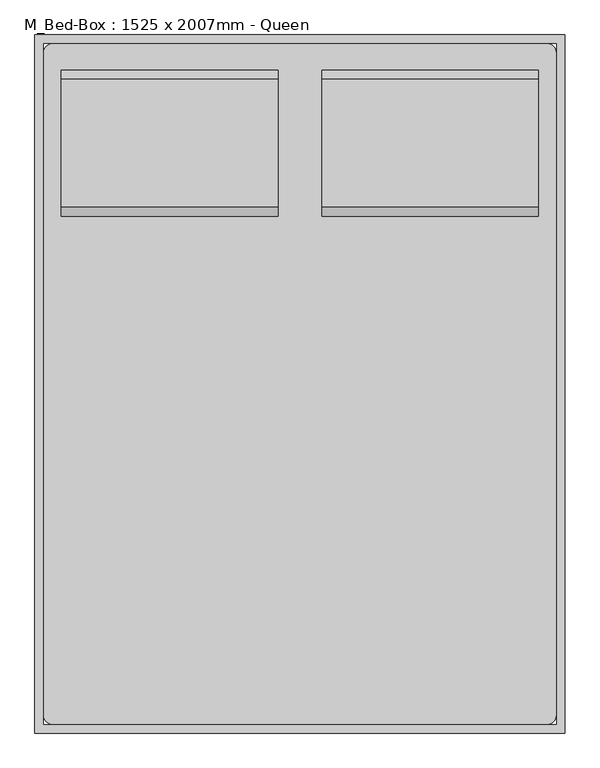
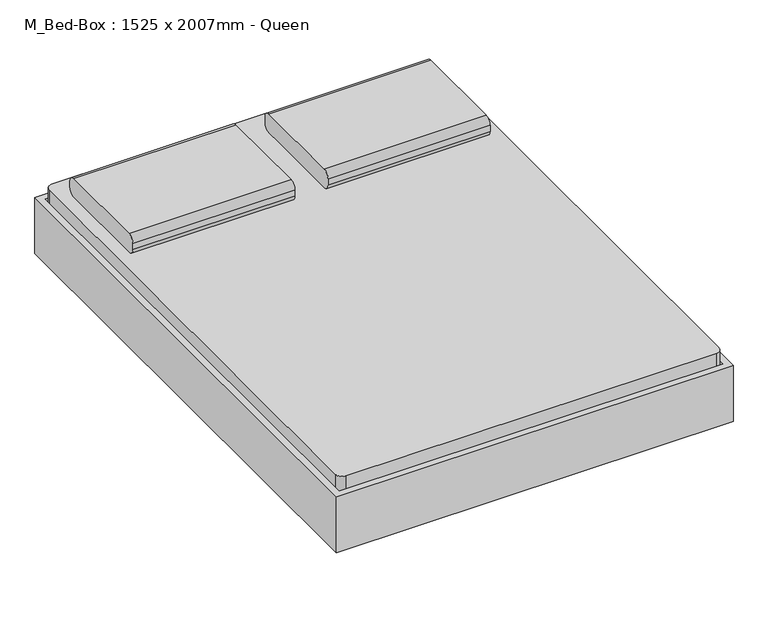
"""IFC4 building model written with IfcOpenShell, lengths in millimetres: furniture geometry, M_Bed-Box : 1525 x 2007mm - Queen."""

import ifcopenshell
import ifcopenshell.guid

model = None  # the IFC model being written
_history = None  # IfcOwnerHistory: only IFC2X3 demands one
_inside = {}  # id of a spatial element -> (the spatial element, [elements in it])
_under = {}  # id of a project, library or spatial element -> (it, [spatial elements below it])
_declared = {}  # id of a project -> (the project, [libraries it declares])
_typed = {}  # id of a type object -> (the type object, [elements of that type])
_made_of = {}  # id of a material, layer set ... -> (it, [elements and type objects made of it])


def new_model(schema):
    """Start an empty IFC model of exactly this schema.

    Asked for "IFC4X3", IfcOpenShell would pick the latest addendum, in which some entities
    have other attributes; the version numbers below select the first issue.
    IFC2X3 requires an IfcOwnerHistory on every rooted entity: one is made here for all.
    """
    global model, _history
    if schema == "IFC4X3":
        model = ifcopenshell.file(schema_version=(4, 3, 0, 0))
    else:
        model = ifcopenshell.file(schema=schema)
    _inside.clear()
    _under.clear()
    _declared.clear()
    _typed.clear()
    _made_of.clear()
    _history = None
    if model.schema == "IFC2X3":
        org = make("IfcOrganization", Name="unknown")
        user = make(
            "IfcPersonAndOrganization",
            ThePerson=make("IfcPerson", FamilyName="unknown"),
            TheOrganization=org,
        )
        app = make(
            "IfcApplication",
            ApplicationDeveloper=org,
            Version="unknown",
            ApplicationFullName="unknown",
            ApplicationIdentifier="unknown",
        )
        _history = make(
            "IfcOwnerHistory",
            OwningUser=user,
            OwningApplication=app,
            ChangeAction="ADDED",
            CreationDate=0,
        )
    return model


def make(cls, **values):
    """One entity of the class cls with the attributes given. An attribute that is None is left unset."""
    return model.create_entity(
        cls, **{name: value for name, value in values.items() if value is not None}
    )


def rooted(cls, **values):
    """An entity with a GlobalId (a new one), such as an element, a storey or a relation."""
    return make(cls, GlobalId=ifcopenshell.guid.new(), OwnerHistory=_history, **values)


def si_unit(unit_type, name, prefix=None):
    """IfcSIUnit, for example si_unit("LENGTHUNIT", "METRE", prefix="MILLI")."""
    return make("IfcSIUnit", UnitType=unit_type, Prefix=prefix, Name=name)


def assignment(units):
    """IfcUnitAssignment: the units of a project."""
    return None if units is None else make("IfcUnitAssignment", Units=units)


def point(xyz):
    """IfcCartesianPoint."""
    return None if xyz is None else make("IfcCartesianPoint", Coordinates=xyz)


def direction(xyz):
    """IfcDirection."""
    return None if xyz is None else make("IfcDirection", DirectionRatios=xyz)


def frame(location, z_axis=None, x_axis=None):
    """IfcAxis2Placement3D, a coordinate frame: its origin and axes. An axis left out is left unset."""
    return make(
        "IfcAxis2Placement3D",
        Location=point(location),
        Axis=direction(z_axis),
        RefDirection=direction(x_axis),
    )


def frame_2d(location, x_axis=None):
    """IfcAxis2Placement2D, a coordinate frame in the plane: its origin and x axis."""
    return make(
        "IfcAxis2Placement2D", Location=point(location), RefDirection=direction(x_axis)
    )


def origin():
    """The frame at (0, 0, 0) with its axes left unset."""
    return frame((0.0, 0.0, 0.0))


def place(relative_to, where):
    """IfcLocalPlacement: puts the frame where relative to a parent placement (None: the world)."""
    return make(
        "IfcLocalPlacement", PlacementRelTo=relative_to, RelativePlacement=where
    )


def context(
    kind, dimensions, precision=None, world=None, true_north=None, identifier=None
):
    """IfcGeometricRepresentationContext, for example the 3D "Model" context."""
    return make(
        "IfcGeometricRepresentationContext",
        ContextIdentifier=identifier,
        ContextType=kind,
        CoordinateSpaceDimension=dimensions,
        Precision=precision,
        WorldCoordinateSystem=world,
        TrueNorth=true_north,
    )


def project(units=None, contexts=None):
    """IfcProject with its units and contexts."""
    return rooted(
        "IfcProject",
        Name="project",
        RepresentationContexts=contexts,
        UnitsInContext=assignment(units),
    )


def spatial(cls, under=None, at=None, **own):
    """A site, building, storey or space (cls), placed at a placement, below another one or the project."""
    s = rooted(cls, ObjectPlacement=at, **own)
    if under is not None:
        _under.setdefault(under.id(), (under, []))[1].append(s)
    return s


def polyline(points):
    """IfcPolyline through the points."""
    return make("IfcPolyline", Points=[point(p) for p in points])


def circle_curve(where, radius):
    """IfcCircle in the frame where."""
    return make("IfcCircle", Position=where, Radius=radius)


def trimmed(basis, trim1, trim2, sense, master):
    """IfcTrimmedCurve: the piece of a basis curve between two trims."""
    return make(
        "IfcTrimmedCurve",
        BasisCurve=basis,
        Trim1=trim1,
        Trim2=trim2,
        SenseAgreement=sense,
        MasterRepresentation=master,
    )


def segment(curve, same_sense, transition):
    """IfcCompositeCurveSegment."""
    return make(
        "IfcCompositeCurveSegment",
        Transition=transition,
        SameSense=same_sense,
        ParentCurve=curve,
    )


def composite_curve(segments, self_intersect=None):
    """IfcCompositeCurve: segments joined end to end."""
    return make("IfcCompositeCurve", Segments=segments, SelfIntersect=self_intersect)


def outline(outer, holes=None, kind="AREA"):
    """IfcArbitraryClosedProfileDef: a profile drawn as a closed curve; with holes, ...WithVoids."""
    if holes is None:
        return make("IfcArbitraryClosedProfileDef", ProfileType=kind, OuterCurve=outer)
    return make(
        "IfcArbitraryProfileDefWithVoids",
        ProfileType=kind,
        OuterCurve=outer,
        InnerCurves=holes,
    )


def extrude(swept, where, along, depth):
    """IfcExtrudedAreaSolid: the profile swept, set in the frame where, extruded along a direction by depth."""
    return make(
        "IfcExtrudedAreaSolid",
        SweptArea=swept,
        Position=where,
        ExtrudedDirection=direction(along),
        Depth=depth,
    )


def shape(context_of_items, identifier, shape_type, items):
    """IfcShapeRepresentation: the items that make up one representation, for example the "Body"."""
    return make(
        "IfcShapeRepresentation",
        ContextOfItems=context_of_items,
        RepresentationIdentifier=identifier,
        RepresentationType=shape_type,
        Items=items,
    )


def source(mapping_origin, context_of_items, identifier, shape_type, items):
    """IfcRepresentationMap: a shape defined once, which mapped items show again and again."""
    return make(
        "IfcRepresentationMap",
        MappingOrigin=mapping_origin,
        MappedRepresentation=shape(context_of_items, identifier, shape_type, items),
    )


def transform(
    local_origin,
    x_axis=None,
    y_axis=None,
    z_axis=None,
    scale=None,
    scale2=None,
    scale3=None,
    uniform=True,
):
    """IfcCartesianTransformationOperator3D, or its non-uniform kind. x_axis, y_axis, z_axis: its Axis1, 2, 3."""
    if uniform:
        return make(
            "IfcCartesianTransformationOperator3D",
            Axis1=direction(x_axis),
            Axis2=direction(y_axis),
            LocalOrigin=point(local_origin),
            Scale=scale,
            Axis3=direction(z_axis),
        )
    return make(
        "IfcCartesianTransformationOperator3DnonUniform",
        Axis1=direction(x_axis),
        Axis2=direction(y_axis),
        LocalOrigin=point(local_origin),
        Scale=scale,
        Axis3=direction(z_axis),
        Scale2=scale2,
        Scale3=scale3,
    )


def mapped(mapping_source, mapping_target):
    """IfcMappedItem: shows the shape of a source again, moved by a transform."""
    return make(
        "IfcMappedItem", MappingSource=mapping_source, MappingTarget=mapping_target
    )


def made_of(thing, what):
    """Note that an element or type object is made of a material, layer set ...; save() writes the relation."""
    if what is not None:
        _made_of.setdefault(what.id(), (what, []))[1].append(thing)
    return thing


def element(
    cls,
    number,
    at=None,
    inside=None,
    cuts=None,
    type_object=None,
    material=None,
    context=None,
    identifier="Body",
    shape_type=None,
    held_by="IfcProductDefinitionShape",
    body=None,
    shapes=None,
    **own,
):
    """One element of the class cls, such as IfcWall. Its Tag is "e" and its number.

    at: its placement. inside: the storey or other place that contains it. cuts: it is an
    opening in that element (IfcRelVoidsElement). A single representation is given by context,
    identifier, shape_type and body (its items); several are given by shapes. held_by: the class
    of the entity that holds the representations. save() writes the other relations.
    """
    e = rooted(cls, Tag="e%d" % number, ObjectPlacement=at, **own)
    if body is not None:
        shapes = [shape(context, identifier, shape_type, body)]
    if shapes is not None:
        e.Representation = make(held_by, Representations=shapes)
    if inside is not None:
        _inside.setdefault(inside.id(), (inside, []))[1].append(e)
    if cuts is not None:
        rooted(
            "IfcRelVoidsElement", RelatingBuildingElement=cuts, RelatedOpeningElement=e
        )
    if type_object is not None:
        _typed.setdefault(type_object.id(), (type_object, []))[1].append(e)
    return made_of(e, material)


def aggregate(whole, parts):
    """IfcRelAggregates: a whole, such as a stair, and the parts it consists of."""
    return rooted("IfcRelAggregates", RelatingObject=whole, RelatedObjects=parts)


def save(model, path):
    """Write the relations noted so far, then the file.

    IfcRelAggregates (storeys below a building ...), IfcRelContainedInSpatialStructure (elements
    in a storey), IfcRelDefinesByType, IfcRelAssociatesMaterial and IfcRelDeclares: one each for
    every whole, place, type object, material and project.
    """
    for whole, parts in _under.values():
        aggregate(whole, parts)
    for where, things in _inside.values():
        rooted(
            "IfcRelContainedInSpatialStructure",
            RelatedElements=things,
            RelatingStructure=where,
        )
    for kind, things in _typed.values():
        rooted("IfcRelDefinesByType", RelatedObjects=things, RelatingType=kind)
    for what, things in _made_of.values():
        rooted("IfcRelAssociatesMaterial", RelatedObjects=things, RelatingMaterial=what)
    for by, libraries in _declared.values():
        rooted("IfcRelDeclares", RelatingContext=by, RelatedDefinitions=libraries)
    model.write(path)


def plane_surface(at):
    """IfcPlane: the flat surface through the origin of the frame at, square to its z axis."""
    return make("IfcPlane", Position=at)


def cylinder_surface(at, radius):
    """IfcCylindricalSurface: all points at the distance radius from the z axis of the frame at."""
    return make("IfcCylindricalSurface", Position=at, Radius=radius)


def revolved_surface(curve, axis_point, axis_direction):
    """IfcSurfaceOfRevolution: the curve turned about the line through axis_point along axis_direction."""
    return make(
        "IfcSurfaceOfRevolution",
        SweptCurve=make("IfcArbitraryOpenProfileDef", ProfileType="CURVE", Curve=curve),
        AxisPosition=make("IfcAxis1Placement", Location=point(axis_point), Axis=direction(axis_direction)),
    )


def advanced_brep(points, edges, surfaces, faces):
    """IfcAdvancedBrep: a solid bounded by faces that lie on surfaces and meet in shared edges.

    An edge is (start, end): straight between two places in points (the first is 0);
    or (start, end, curve); or (start, end, curve, False) where it runs against its curve.
    A face is (place in surfaces, loops), or (place, loops, False) where it looks against
    its surface's normal. A loop lists edges by number (the first is 1), with a minus sign
    where the edge is run from its end to its start. The first loop is the outer one.
    """
    corners = [point(p) for p in points]
    vertices = [make("IfcVertexPoint", VertexGeometry=c) for c in corners]
    made = []
    for start, end, *more in edges:
        made.append(
            make(
                "IfcEdgeCurve",
                EdgeStart=vertices[start],
                EdgeEnd=vertices[end],
                EdgeGeometry=more[0] if more else make("IfcPolyline", Points=[corners[start], corners[end]]),
                SameSense=more[1] if len(more) > 1 else True,
            )
        )
    hull = []
    for where, loops, *sense in faces:
        bounds = []
        for j, loop in enumerate(loops):
            ring = [make("IfcOrientedEdge", EdgeElement=made[abs(k) - 1], Orientation=k > 0) for k in loop]
            bounds.append(
                make(
                    "IfcFaceOuterBound" if j == 0 else "IfcFaceBound",
                    Bound=make("IfcEdgeLoop", EdgeList=ring),
                    Orientation=True,
                )
            )
        hull.append(make("IfcAdvancedFace", Bounds=bounds, FaceSurface=surfaces[where], SameSense=sense[0] if sense else True))
    return make("IfcAdvancedBrep", Outer=make("IfcClosedShell", CfsFaces=hull))


def m_bed_box_1525_x_2007mm_queen_e2603687(model_context):
    return source(origin(), model_context, "Body", "SolidModel", [
        extrude(outline(composite_curve([segment(polyline([(642.0704918, 406.4), (273.7704918, 406.4)]), True, "CONTINUOUS"), segment(trimmed(circle_curve(frame_2d((273.7704918, 431.8)), 25.4), [point((273.7704918, 406.4))], [point((248.3704918, 431.8))], False, "CARTESIAN"), True, "CONTINUOUS"), segment(polyline([(248.3704918, 431.8), (248.3704918, 457.2)]), True, "CONTINUOUS"), segment(trimmed(circle_curve(frame_2d((273.7704918, 457.2)), 25.4), [point((248.3704918, 457.2))], [point((273.7704918, 482.6))], False, "CARTESIAN"), True, "CONTINUOUS"), segment(polyline([(273.7704918, 482.6), (642.0704918, 482.6)]), True, "CONTINUOUS"), segment(trimmed(circle_curve(frame_2d((642.0704918, 457.2)), 25.4), [point((642.0704918, 482.6))], [point((667.4704918, 457.2))], False, "CARTESIAN"), True, "CONTINUOUS"), segment(polyline([(667.4704918, 457.2), (667.4704918, 431.8)]), True, "CONTINUOUS"), segment(trimmed(circle_curve(frame_2d((642.0704918, 431.8)), 25.4), [point((667.4704918, 431.8))], [point((642.0704918, 406.4))], False, "CARTESIAN"), True, "CONTINUOUS")], self_intersect=False)), frame((402.652459, 0.0, 0.0), z_axis=(1.0, 0.0, 0.0), x_axis=(0.0, 1.0, 0.0)), (0.0, 0.0, 1.0), 622.8),
        extrude(outline(composite_curve([segment(polyline([(642.0704918, 406.4), (273.7704918, 406.4)]), True, "CONTINUOUS"), segment(trimmed(circle_curve(frame_2d((273.7704918, 431.8)), 25.4), [point((273.7704918, 406.4))], [point((248.3704918, 431.8))], False, "CARTESIAN"), True, "CONTINUOUS"), segment(polyline([(248.3704918, 431.8), (248.3704918, 457.2)]), True, "CONTINUOUS"), segment(trimmed(circle_curve(frame_2d((273.7704918, 457.2)), 25.4), [point((248.3704918, 457.2))], [point((273.7704918, 482.6))], False, "CARTESIAN"), True, "CONTINUOUS"), segment(polyline([(273.7704918, 482.6), (642.0704918, 482.6)]), True, "CONTINUOUS"), segment(trimmed(circle_curve(frame_2d((642.0704918, 457.2)), 25.4), [point((642.0704918, 482.6))], [point((667.4704918, 457.2))], False, "CARTESIAN"), True, "CONTINUOUS"), segment(polyline([(667.4704918, 457.2), (667.4704918, 431.8)]), True, "CONTINUOUS"), segment(trimmed(circle_curve(frame_2d((642.0704918, 431.8)), 25.4), [point((667.4704918, 431.8))], [point((642.0704918, 406.4))], False, "CARTESIAN"), True, "CONTINUOUS")], self_intersect=False)), frame((-347.147541, 0.0, 0.0), z_axis=(1.0, 0.0, 0.0), x_axis=(0.0, 1.0, 0.0)), (0.0, 0.0, 1.0), 622.8),
        advanced_brep(
        [(-397.6231784, 515.0704918, 177.8), (-397.6231784, 438.8704918, 177.8), (-397.6231784, 438.8704918, 196.85), (-397.6231784, 515.0704918, 196.85), (-346.8231784, 515.0704918, 177.8), (-346.8231784, 438.8704918, 177.8), (-334.6869899, 438.8704918, 196.85), (-334.6869899, 515.0704918, 196.85), (-270.7523099, 515.0704918, 14.6654962), (-270.7523099, 438.8704918, 14.6654962), (-253.4871466, 438.8704918, 22.716374), (-253.4871466, 515.0704918, 22.716374), (-247.7320921, 438.8704918, 0.0), (-247.7320921, 515.0704918, 0.0), (-247.7320921, 438.8704918, 19.05), (-247.7320921, 515.0704918, 19.05), (-169.1195862, 515.0704918, 0.0), (-169.1195862, 438.8704918, 0.0), (-169.1195862, 438.8704918, 19.05), (-169.1195862, 515.0704918, 19.05), (-156.4195862, 438.8704918, 3.4029547), (-156.4195862, 515.0704918, 3.4029547), (-165.9445862, 438.8704918, 19.9007387), (-165.9445862, 515.0704918, 19.9007387), (-96.322541, 515.0704918, 38.1), (-96.322541, 438.8704918, 38.1), (-101.4269731, 438.8704918, 57.15), (-101.4269731, 515.0704918, 57.15), (774.9518216, 515.0704918, 38.1), (774.9518216, 438.8704918, 38.1), (780.0562537, 438.8704918, 57.15), (780.0562537, 515.0704918, 57.15), (835.0488669, 515.0704918, 3.4029547), (835.0488669, 438.8704918, 3.4029547), (844.5738669, 438.8704918, 19.9007387), (844.5738669, 515.0704918, 19.9007387), (847.7488669, 438.8704918, 0.0), (847.7488669, 515.0704918, 0.0), (847.7488669, 438.8704918, 19.05), (847.7488669, 515.0704918, 19.05), (926.3613728, 515.0704918, 0.0), (926.3613728, 438.8704918, 0.0), (926.3613728, 438.8704918, 19.05), (926.3613728, 515.0704918, 19.05), (949.3815906, 438.8704918, 14.6654962), (949.3815906, 515.0704918, 14.6654962), (932.1164272, 438.8704918, 22.716374), (932.1164272, 515.0704918, 22.716374), (1025.452459, 515.0704918, 177.8), (1025.452459, 438.8704918, 177.8), (1013.3162705, 438.8704918, 196.85), (1013.3162705, 515.0704918, 196.85), (1076.252459, 515.0704918, 177.8), (1076.252459, 515.0704918, 196.85), (1076.252459, 438.8704918, 196.85), (1076.252459, 438.8704918, 177.8)],
        [
            (0, 1),
            (1, 2),
            (2, 3),
            (3, 0),
            (0, 4),
            (4, 5),
            (5, 1),
            (5, 6),
            (6, 2),
            (6, 7),
            (7, 3),
            (7, 4),
            (4, 8),
            (8, 9),
            (9, 5),
            (9, 10),
            (10, 6),
            (10, 11),
            (11, 7),
            (11, 8),
            (12, 9, circle_curve(frame((-247.7320921, 438.8704918, 25.4), z_axis=(0.0, 1.0, 0.0), x_axis=(-0.906307787036649, 0.0, -0.4226182617407015)), 25.4)),
            (8, 13, circle_curve(frame((-247.7320921, 515.0704918, 25.4), z_axis=(0.0, -1.0, 0.0), x_axis=(-0.906307787036649, 0.0, -0.4226182617407015)), 25.4)),
            (13, 12),
            (14, 10, circle_curve(frame((-247.7320921, 438.8704918, 25.4), z_axis=(0.0, 1.0, 0.0), x_axis=(-0.906307787036649, 0.0, -0.4226182617407015)), 6.35)),
            (12, 14),
            (15, 11, circle_curve(frame((-247.7320921, 515.0704918, 25.4), z_axis=(0.0, 1.0, 0.0), x_axis=(-0.906307787036649, 0.0, -0.4226182617407015)), 6.35)),
            (14, 15),
            (15, 13),
            (13, 16),
            (16, 17),
            (17, 12),
            (17, 18),
            (18, 14),
            (18, 19),
            (19, 15),
            (19, 16),
            (20, 17, circle_curve(frame((-169.1195862, 438.8704918, 25.4), z_axis=(0.0, 1.0, 0.0), x_axis=(0.0, 0.0, -1.0)), 25.4)),
            (16, 21, circle_curve(frame((-169.1195862, 515.0704918, 25.4), z_axis=(0.0, -1.0, 0.0), x_axis=(0.0, 0.0, -1.0)), 25.4)),
            (21, 20),
            (22, 18, circle_curve(frame((-169.1195862, 438.8704918, 25.4), z_axis=(0.0, 1.0, 0.0), x_axis=(0.0, 0.0, -1.0)), 6.35)),
            (20, 22),
            (23, 19, circle_curve(frame((-169.1195862, 515.0704918, 25.4), z_axis=(0.0, 1.0, 0.0), x_axis=(0.0, 0.0, -1.0)), 6.35)),
            (22, 23),
            (23, 21),
            (21, 24),
            (24, 25),
            (25, 20),
            (25, 26),
            (26, 22),
            (26, 27),
            (27, 23),
            (27, 24),
            (24, 28),
            (28, 29),
            (29, 25),
            (29, 30),
            (30, 26),
            (30, 31),
            (31, 27),
            (31, 28),
            (28, 32),
            (32, 33),
            (33, 29),
            (33, 34),
            (34, 30),
            (34, 35),
            (35, 31),
            (35, 32),
            (36, 33, circle_curve(frame((847.7488669, 438.8704918, 25.4), z_axis=(0.0, 1.0, 0.0), x_axis=(-0.5000000000000463, 0.0, -0.8660254037844118)), 25.4)),
            (32, 37, circle_curve(frame((847.7488669, 515.0704918, 25.4), z_axis=(0.0, -1.0, 0.0), x_axis=(-0.5000000000000463, 0.0, -0.8660254037844118)), 25.4)),
            (37, 36),
            (38, 34, circle_curve(frame((847.7488669, 438.8704918, 25.4), z_axis=(0.0, 1.0, 0.0), x_axis=(-0.5000000000000463, 0.0, -0.8660254037844118)), 6.35)),
            (36, 38),
            (39, 35, circle_curve(frame((847.7488669, 515.0704918, 25.4), z_axis=(0.0, 1.0, 0.0), x_axis=(-0.5000000000000463, 0.0, -0.8660254037844118)), 6.35)),
            (38, 39),
            (39, 37),
            (37, 40),
            (40, 41),
            (41, 36),
            (41, 42),
            (42, 38),
            (42, 43),
            (43, 39),
            (43, 40),
            (44, 41, circle_curve(frame((926.3613728, 438.8704918, 25.4), z_axis=(0.0, 1.0, 0.0), x_axis=(0.0, 0.0, -1.0)), 25.4)),
            (40, 45, circle_curve(frame((926.3613728, 515.0704918, 25.4), z_axis=(0.0, -1.0, 0.0), x_axis=(0.0, 0.0, -1.0)), 25.4)),
            (45, 44),
            (46, 42, circle_curve(frame((926.3613728, 438.8704918, 25.4), z_axis=(0.0, 1.0, 0.0), x_axis=(0.0, 0.0, -1.0)), 6.35)),
            (44, 46),
            (47, 43, circle_curve(frame((926.3613728, 515.0704918, 25.4), z_axis=(0.0, 1.0, 0.0), x_axis=(0.0, 0.0, -1.0)), 6.35)),
            (46, 47),
            (47, 45),
            (45, 48),
            (48, 49),
            (49, 44),
            (49, 50),
            (50, 46),
            (50, 51),
            (51, 47),
            (51, 48),
            (52, 53),
            (53, 54),
            (54, 55),
            (55, 52),
            (48, 52),
            (55, 49),
            (54, 50),
            (53, 51),
        ],
        [
            plane_surface(frame((-397.6231784, 769.0704918, -152.9490627), z_axis=(-1.0, 0.0, 0.0), x_axis=(0.0, 1.0, 0.0))),
            plane_surface(frame((-397.6231784, 515.0704918, 177.8), z_axis=(0.0, 0.0, -1.0), x_axis=(1.0, 0.0, 0.0))),
            plane_surface(frame((-397.6231784, 438.8704918, 177.8), z_axis=(0.0, -1.0, 0.0), x_axis=(1.0, 0.0, 0.0))),
            plane_surface(frame((-397.6231784, 438.8704918, 196.85), z_axis=(0.0, 0.0, 1.0), x_axis=(1.0, 0.0, 0.0))),
            plane_surface(frame((-397.6231784, 515.0704918, 196.85), z_axis=(0.0, 1.0, 0.0), x_axis=(1.0, 0.0, 0.0))),
            plane_surface(frame((-346.8231784, 515.0704918, 177.8), z_axis=(-0.9063077870366485, 0.0, -0.4226182617407029), x_axis=(0.4226182617407029, 0.0, -0.9063077870366485))),
            plane_surface(frame((-346.8231784, 438.8704918, 177.8), z_axis=(0.0, -1.0, 0.0), x_axis=(0.42261826174070266, 0.0, -0.9063077870366485))),
            plane_surface(frame((-334.6869899, 438.8704918, 196.85), z_axis=(0.9063077870366486, 0.0, 0.4226182617407026), x_axis=(0.4226182617407026, 0.0, -0.9063077870366486))),
            plane_surface(frame((-334.6869899, 515.0704918, 196.85), z_axis=(0.0, 1.0, 0.0), x_axis=(0.42261826174070266, 0.0, -0.9063077870366485))),
            cylinder_surface(frame((-247.7320921, 769.0704918, 25.4), z_axis=(0.0, -1.0, 0.0), x_axis=(-0.906307787036649, 0.0, -0.4226182617407015)), 25.4),
            plane_surface(frame((-247.7320921, 438.8704918, 25.4), z_axis=(0.0, -1.0, 0.0), x_axis=(-0.906307787036649, 0.0, -0.4226182617407015))),
            revolved_surface(polyline([(-253.4871465476827, 438.8704918, 22.716374037946544), (-253.4871465476827, 515.0704918, 22.716374037946544)]), (-247.7320921, 769.0704918, 25.4), (0.0, -1.0, 0.0)),
            plane_surface(frame((-247.7320921, 515.0704918, 25.4), z_axis=(0.0, 1.0, 0.0), x_axis=(-0.906307787036649, 0.0, -0.4226182617407015))),
            plane_surface(frame((-247.7320921, 515.0704918, 0.0), z_axis=(0.0, 0.0, -1.0), x_axis=(1.0, 0.0, 0.0))),
            plane_surface(frame((-247.7320921, 438.8704918, 0.0), z_axis=(0.0, -1.0, 0.0), x_axis=(1.0, 0.0, 0.0))),
            plane_surface(frame((-247.7320921, 438.8704918, 19.05), z_axis=(0.0, 0.0, 1.0), x_axis=(1.0, 0.0, 0.0))),
            plane_surface(frame((-247.7320921, 515.0704918, 19.05), z_axis=(0.0, 1.0, 0.0), x_axis=(1.0, 0.0, 0.0))),
            cylinder_surface(frame((-169.1195862, 769.0704918, 25.4), z_axis=(0.0, -1.0, 0.0), x_axis=(0.0, 0.0, -1.0)), 25.4),
            plane_surface(frame((-169.1195862, 438.8704918, 25.4), z_axis=(0.0, -1.0, 0.0), x_axis=(0.0, 0.0, -1.0))),
            revolved_surface(polyline([(-169.1195862, 438.8704918, 19.049999999999997), (-169.1195862, 515.0704918, 19.049999999999997)]), (-169.1195862, 769.0704918, 25.4), (0.0, -1.0, 0.0)),
            plane_surface(frame((-169.1195862, 515.0704918, 25.4), z_axis=(0.0, 1.0, 0.0), x_axis=(0.0, 0.0, -1.0))),
            plane_surface(frame((-156.4195862, 515.0704918, 3.4029547), z_axis=(0.49999999999987765, 0.0, -0.8660254037845093), x_axis=(0.8660254037845093, 0.0, 0.49999999999987765))),
            plane_surface(frame((-156.4195862, 438.8704918, 3.4029547), z_axis=(0.0, -1.0, 0.0), x_axis=(0.8660254037845091, 0.0, 0.499999999999878))),
            plane_surface(frame((-165.9445862, 438.8704918, 19.9007387), z_axis=(-0.49999999999987765, 0.0, 0.8660254037845093), x_axis=(0.8660254037845093, 0.0, 0.49999999999987765))),
            plane_surface(frame((-165.9445862, 515.0704918, 19.9007387), z_axis=(0.0, 1.0000000000000002, 0.0), x_axis=(0.8660254037845089, 0.0, 0.4999999999998785))),
            plane_surface(frame((-96.322541, 515.0704918, 38.1), z_axis=(0.0, 0.0, -1.0), x_axis=(1.0, 0.0, 0.0))),
            plane_surface(frame((-96.322541, 438.8704918, 38.1), z_axis=(0.0, -1.0, 0.0), x_axis=(1.0, 0.0, 0.0))),
            plane_surface(frame((-101.4269731, 438.8704918, 57.15), z_axis=(0.0, 0.0, 1.0), x_axis=(1.0, 0.0, 0.0))),
            plane_surface(frame((-101.4269731, 515.0704918, 57.15), z_axis=(0.0, 1.0, 0.0), x_axis=(1.0, 0.0, 0.0))),
            plane_surface(frame((774.9518216, 515.0704918, 38.1), z_axis=(-0.5000000000000452, 0.0, -0.8660254037844126), x_axis=(0.8660254037844126, 0.0, -0.5000000000000452))),
            plane_surface(frame((774.9518216, 438.8704918, 38.1), z_axis=(0.0, -1.0, 0.0), x_axis=(0.8660254037844124, 0.0, -0.5000000000000455))),
            plane_surface(frame((780.0562537, 438.8704918, 57.15), z_axis=(0.5000000000000464, 0.0, 0.8660254037844118), x_axis=(0.8660254037844118, 0.0, -0.5000000000000464))),
            plane_surface(frame((780.0562537, 515.0704918, 57.15), z_axis=(0.0, 1.0000000000000002, 0.0), x_axis=(0.866025403784413, 0.0, -0.5000000000000447))),
            cylinder_surface(frame((847.7488669, 769.0704918, 25.4), z_axis=(0.0, -1.0, 0.0), x_axis=(-0.5000000000000463, 0.0, -0.8660254037844118)), 25.4),
            plane_surface(frame((847.7488669, 438.8704918, 25.4), z_axis=(0.0, -1.0000000000000002, 0.0), x_axis=(-0.5000000000000464, 0.0, -0.866025403784412))),
            revolved_surface(polyline([(844.5738668999998, 438.8704918, 19.90073868596898), (844.5738668999998, 515.0704918, 19.90073868596898)]), (847.7488669, 769.0704918, 25.4), (0.0, -1.0, 0.0)),
            plane_surface(frame((847.7488669, 515.0704918, 25.4), z_axis=(0.0, 1.0000000000000002, 0.0), x_axis=(-0.5000000000000464, 0.0, -0.866025403784412))),
            plane_surface(frame((847.7488669, 515.0704918, 0.0), z_axis=(0.0, 0.0, -1.0), x_axis=(1.0, 0.0, 0.0))),
            plane_surface(frame((847.7488669, 438.8704918, 0.0), z_axis=(0.0, -1.0, 0.0), x_axis=(1.0, 0.0, 0.0))),
            plane_surface(frame((847.7488669, 438.8704918, 19.05), z_axis=(0.0, 0.0, 1.0), x_axis=(1.0, 0.0, 0.0))),
            plane_surface(frame((847.7488669, 515.0704918, 19.05), z_axis=(0.0, 1.0, 0.0), x_axis=(1.0, 0.0, 0.0))),
            cylinder_surface(frame((926.3613728, 769.0704918, 25.4), z_axis=(0.0, -1.0, 0.0), x_axis=(0.0, 0.0, -1.0)), 25.4),
            plane_surface(frame((926.3613728, 438.8704918, 25.4), z_axis=(0.0, -1.0, 0.0), x_axis=(0.0, 0.0, -1.0))),
            revolved_surface(polyline([(926.3613728, 438.8704918, 19.049999999999997), (926.3613728, 515.0704918, 19.049999999999997)]), (926.3613728, 769.0704918, 25.4), (0.0, -1.0, 0.0)),
            plane_surface(frame((926.3613728, 515.0704918, 25.4), z_axis=(0.0, 1.0, 0.0), x_axis=(0.0, 0.0, -1.0))),
            plane_surface(frame((949.3815906, 515.0704918, 14.6654962), z_axis=(0.9063077870366805, 0.0, -0.422618261740634), x_axis=(0.422618261740634, 0.0, 0.9063077870366805))),
            plane_surface(frame((949.3815906, 438.8704918, 14.6654962), z_axis=(0.0, -1.0, 0.0), x_axis=(0.4226182617406339, 0.0, 0.9063077870366806))),
            plane_surface(frame((932.1164272, 438.8704918, 22.716374), z_axis=(-0.9063077870366808, 0.0, 0.4226182617406335), x_axis=(0.4226182617406335, 0.0, 0.9063077870366808))),
            plane_surface(frame((932.1164272, 515.0704918, 22.716374), z_axis=(0.0, 1.0, 0.0), x_axis=(0.42261826174063294, 0.0, 0.906307787036681))),
            plane_surface(frame((1076.252459, 769.0704918, -152.9490627), z_axis=(1.0, 0.0, 0.0), x_axis=(0.0, 1.0, 0.0))),
            plane_surface(frame((1025.452459, 515.0704918, 177.8), z_axis=(0.0, 0.0, -1.0), x_axis=(1.0, 0.0, 0.0))),
            plane_surface(frame((1025.452459, 438.8704918, 177.8), z_axis=(0.0, -1.0, 0.0), x_axis=(1.0, 0.0, 0.0))),
            plane_surface(frame((1013.3162705, 438.8704918, 196.85), z_axis=(0.0, 0.0, 1.0), x_axis=(1.0, 0.0, 0.0))),
            plane_surface(frame((1013.3162705, 515.0704918, 196.85), z_axis=(0.0, 1.0, 0.0), x_axis=(1.0, 0.0, 0.0))),
        ],
        [
            (0, [[1, 2, 3, 4]]),
            (1, [[-1, 5, 6, 7]]),
            (2, [[-2, -7, 8, 9]]),
            (3, [[-3, -9, 10, 11]]),
            (4, [[-4, -11, 12, -5]]),
            (5, [[-6, 13, 14, 15]]),
            (6, [[-8, -15, 16, 17]]),
            (7, [[-10, -17, 18, 19]]),
            (8, [[-12, -19, 20, -13]]),
            (9, [[21, -14, 22, 23]]),
            (10, [[24, -16, -21, 25]]),
            (11, [[26, -18, -24, 27]]),
            (12, [[-22, -20, -26, 28]]),
            (13, [[-23, 29, 30, 31]]),
            (14, [[-25, -31, 32, 33]]),
            (15, [[-27, -33, 34, 35]]),
            (16, [[-28, -35, 36, -29]]),
            (17, [[37, -30, 38, 39]]),
            (18, [[40, -32, -37, 41]]),
            (19, [[42, -34, -40, 43]]),
            (20, [[-38, -36, -42, 44]]),
            (21, [[-39, 45, 46, 47]]),
            (22, [[-41, -47, 48, 49]]),
            (23, [[-43, -49, 50, 51]]),
            (24, [[-44, -51, 52, -45]]),
            (25, [[-46, 53, 54, 55]]),
            (26, [[-48, -55, 56, 57]]),
            (27, [[-50, -57, 58, 59]]),
            (28, [[-52, -59, 60, -53]]),
            (29, [[-54, 61, 62, 63]]),
            (30, [[-56, -63, 64, 65]]),
            (31, [[-58, -65, 66, 67]]),
            (32, [[-60, -67, 68, -61]]),
            (33, [[69, -62, 70, 71]]),
            (34, [[72, -64, -69, 73]]),
            (35, [[74, -66, -72, 75]]),
            (36, [[-70, -68, -74, 76]]),
            (37, [[-71, 77, 78, 79]]),
            (38, [[-73, -79, 80, 81]]),
            (39, [[-75, -81, 82, 83]]),
            (40, [[-76, -83, 84, -77]]),
            (41, [[85, -78, 86, 87]]),
            (42, [[88, -80, -85, 89]]),
            (43, [[90, -82, -88, 91]]),
            (44, [[-86, -84, -90, 92]]),
            (45, [[-87, 93, 94, 95]]),
            (46, [[-89, -95, 96, 97]]),
            (47, [[-91, -97, 98, 99]]),
            (48, [[-92, -99, 100, -93]]),
            (49, [[101, 102, 103, 104]]),
            (50, [[-94, 105, -104, 106]]),
            (51, [[-96, -106, -103, 107]]),
            (52, [[-98, -107, -102, 108]]),
            (53, [[-100, -108, -101, -105]]),
        ],
    ),
        extrude(outline(composite_curve([segment(polyline([(-372.547541, 743.6704918), (1050.852459, 743.6704918)]), True, "CONTINUOUS"), segment(trimmed(circle_curve(frame_2d((1050.852459, 718.2704918)), 25.4), [point((1050.852459, 743.6704918))], [point((1076.252459, 718.2704918))], False, "CARTESIAN"), True, "CONTINUOUS"), segment(polyline([(1076.252459, 718.2704918), (1076.252459, -1187.1295082)]), True, "CONTINUOUS"), segment(trimmed(circle_curve(frame_2d((1050.852459, -1187.1295082)), 25.4), [point((1076.252459, -1187.1295082))], [point((1050.852459, -1212.5295082))], False, "CARTESIAN"), True, "CONTINUOUS"), segment(polyline([(1050.852459, -1212.5295082), (-372.547541, -1212.5295082)]), True, "CONTINUOUS"), segment(trimmed(circle_curve(frame_2d((-372.547541, -1187.1295082)), 25.4), [point((-372.547541, -1212.5295082))], [point((-397.947541, -1187.1295082))], False, "CARTESIAN"), True, "CONTINUOUS"), segment(polyline([(-397.947541, -1187.1295082), (-397.947541, 718.2704918)]), True, "CONTINUOUS"), segment(trimmed(circle_curve(frame_2d((-372.547541, 718.2704918)), 25.4), [point((-397.947541, 718.2704918))], [point((-372.547541, 743.6704918))], False, "CARTESIAN"), True, "CONTINUOUS")], self_intersect=False)), frame((0.0, 0.0, 203.2), z_axis=(0.0, 0.0, 1.0), x_axis=(1.0, 0.0, 0.0)), (0.0, 0.0, 1.0), 203.2),
        advanced_brep(
        [(-397.947541, -933.1295082, 196.85), (-397.947541, -933.1295082, 177.8), (-397.947541, -1009.3295082, 177.8), (-397.947541, -1009.3295082, 196.85), (-335.0113525, -933.1295082, 196.85), (-347.147541, -933.1295082, 177.8), (-347.147541, -1009.3295082, 177.8), (-335.0113525, -1009.3295082, 196.85), (-253.8115092, -933.1295082, 22.716374), (-271.0766725, -933.1295082, 14.6654962), (-271.0766725, -1009.3295082, 14.6654962), (-253.8115092, -1009.3295082, 22.716374), (-248.0564547, -933.1295082, 0.0), (-248.0564547, -933.1295082, 19.05), (-248.0564547, -1009.3295082, 0.0), (-248.0564547, -1009.3295082, 19.05), (-169.4439489, -933.1295082, 19.05), (-169.4439489, -933.1295082, 0.0), (-169.4439489, -1009.3295082, 0.0), (-169.4439489, -1009.3295082, 19.05), (-156.7439489, -933.1295082, 3.4029547), (-166.2689489, -933.1295082, 19.9007387), (-156.7439489, -1009.3295082, 3.4029547), (-166.2689489, -1009.3295082, 19.9007387), (-101.7513357, -933.1295082, 57.15), (-96.6469036, -933.1295082, 38.1), (-96.6469036, -1009.3295082, 38.1), (-101.7513357, -1009.3295082, 57.15), (780.0562537, -933.1295082, 57.15), (774.9518216, -933.1295082, 38.1), (774.9518216, -1009.3295082, 38.1), (780.0562537, -1009.3295082, 57.15), (844.5738669, -933.1295082, 19.9007387), (835.0488669, -933.1295082, 3.4029547), (835.0488669, -1009.3295082, 3.4029547), (844.5738669, -1009.3295082, 19.9007387), (847.7488669, -933.1295082, 0.0), (847.7488669, -933.1295082, 19.05), (847.7488669, -1009.3295082, 0.0), (847.7488669, -1009.3295082, 19.05), (926.3613728, -933.1295082, 19.05), (926.3613728, -933.1295082, 0.0), (926.3613728, -1009.3295082, 0.0), (926.3613728, -1009.3295082, 19.05), (949.3815906, -933.1295082, 14.6654962), (932.1164272, -933.1295082, 22.716374), (949.3815906, -1009.3295082, 14.6654962), (932.1164272, -1009.3295082, 22.716374), (1013.3162705, -933.1295082, 196.85), (1025.452459, -933.1295082, 177.8), (1025.452459, -1009.3295082, 177.8), (1013.3162705, -1009.3295082, 196.85), (1076.252459, -933.1295082, 196.85), (1076.252459, -1009.3295082, 196.85), (1076.252459, -1009.3295082, 177.8), (1076.252459, -933.1295082, 177.8)],
        [
            (0, 1),
            (1, 2),
            (2, 3),
            (3, 0),
            (0, 4),
            (4, 5),
            (5, 1),
            (5, 6),
            (6, 2),
            (6, 7),
            (7, 3),
            (7, 4),
            (4, 8),
            (8, 9),
            (9, 5),
            (9, 10),
            (10, 6),
            (10, 11),
            (11, 7),
            (11, 8),
            (12, 9, circle_curve(frame((-248.0564547, -933.1295082, 25.4), z_axis=(0.0, 1.0, 0.0), x_axis=(-0.9063077870366625, 0.0, -0.4226182617406725)), 25.4)),
            (8, 13, circle_curve(frame((-248.0564547, -933.1295082, 25.4), z_axis=(0.0, -1.0, 0.0), x_axis=(-0.9063077870366625, 0.0, -0.4226182617406725)), 6.35)),
            (13, 12),
            (14, 10, circle_curve(frame((-248.0564547, -1009.3295082, 25.4), z_axis=(0.0, 1.0, 0.0), x_axis=(-0.9063077870366625, 0.0, -0.4226182617406725)), 25.4)),
            (12, 14),
            (15, 11, circle_curve(frame((-248.0564547, -1009.3295082, 25.4), z_axis=(0.0, 1.0, 0.0), x_axis=(-0.9063077870366625, 0.0, -0.4226182617406725)), 6.35)),
            (14, 15),
            (15, 13),
            (13, 16),
            (16, 17),
            (17, 12),
            (17, 18),
            (18, 14),
            (18, 19),
            (19, 15),
            (19, 16),
            (20, 17, circle_curve(frame((-169.4439489, -933.1295082, 25.4), z_axis=(0.0, 1.0, 0.0), x_axis=(0.0, 0.0, -1.0)), 25.4)),
            (16, 21, circle_curve(frame((-169.4439489, -933.1295082, 25.4), z_axis=(0.0, -1.0, 0.0), x_axis=(0.0, 0.0, -1.0)), 6.35)),
            (21, 20),
            (22, 18, circle_curve(frame((-169.4439489, -1009.3295082, 25.4), z_axis=(0.0, 1.0, 0.0), x_axis=(0.0, 0.0, -1.0)), 25.4)),
            (20, 22),
            (23, 19, circle_curve(frame((-169.4439489, -1009.3295082, 25.4), z_axis=(0.0, 1.0, 0.0), x_axis=(0.0, 0.0, -1.0)), 6.35)),
            (22, 23),
            (23, 21),
            (21, 24),
            (24, 25),
            (25, 20),
            (25, 26),
            (26, 22),
            (26, 27),
            (27, 23),
            (27, 24),
            (24, 28),
            (28, 29),
            (29, 25),
            (29, 30),
            (30, 26),
            (30, 31),
            (31, 27),
            (31, 28),
            (28, 32),
            (32, 33),
            (33, 29),
            (33, 34),
            (34, 30),
            (34, 35),
            (35, 31),
            (35, 32),
            (36, 33, circle_curve(frame((847.7488669, -933.1295082, 25.4), z_axis=(0.0, 1.0, 0.0), x_axis=(-0.5000000000000528, 0.0, -0.8660254037844081)), 25.4)),
            (32, 37, circle_curve(frame((847.7488669, -933.1295082, 25.4), z_axis=(0.0, -1.0, 0.0), x_axis=(-0.5000000000000528, 0.0, -0.8660254037844081)), 6.35)),
            (37, 36),
            (38, 34, circle_curve(frame((847.7488669, -1009.3295082, 25.4), z_axis=(0.0, 1.0, 0.0), x_axis=(-0.5000000000000528, 0.0, -0.8660254037844081)), 25.4)),
            (36, 38),
            (39, 35, circle_curve(frame((847.7488669, -1009.3295082, 25.4), z_axis=(0.0, 1.0, 0.0), x_axis=(-0.5000000000000528, 0.0, -0.8660254037844081)), 6.35)),
            (38, 39),
            (39, 37),
            (37, 40),
            (40, 41),
            (41, 36),
            (41, 42),
            (42, 38),
            (42, 43),
            (43, 39),
            (43, 40),
            (44, 41, circle_curve(frame((926.3613728, -933.1295082, 25.4), z_axis=(0.0, 1.0, 0.0), x_axis=(0.0, 0.0, -1.0)), 25.4)),
            (40, 45, circle_curve(frame((926.3613728, -933.1295082, 25.4), z_axis=(0.0, -1.0, 0.0), x_axis=(0.0, 0.0, -1.0)), 6.35)),
            (45, 44),
            (46, 42, circle_curve(frame((926.3613728, -1009.3295082, 25.4), z_axis=(0.0, 1.0, 0.0), x_axis=(0.0, 0.0, -1.0)), 25.4)),
            (44, 46),
            (47, 43, circle_curve(frame((926.3613728, -1009.3295082, 25.4), z_axis=(0.0, 1.0, 0.0), x_axis=(0.0, 0.0, -1.0)), 6.35)),
            (46, 47),
            (47, 45),
            (45, 48),
            (48, 49),
            (49, 44),
            (49, 50),
            (50, 46),
            (50, 51),
            (51, 47),
            (51, 48),
            (52, 53),
            (53, 54),
            (54, 55),
            (55, 52),
            (48, 52),
            (55, 49),
            (54, 50),
            (53, 51),
        ],
        [
            plane_surface(frame((-397.947541, -1237.9295082, -127.5947323), z_axis=(-1.0, 0.0, 0.0), x_axis=(0.0, 1.0, 0.0))),
            plane_surface(frame((-397.947541, -933.1295082, 196.85), z_axis=(0.0, 1.0, 0.0), x_axis=(1.0, 0.0, 0.0))),
            plane_surface(frame((-397.947541, -933.1295082, 177.8), z_axis=(0.0, 0.0, -1.0), x_axis=(1.0, 0.0, 0.0))),
            plane_surface(frame((-397.947541, -1009.3295082, 177.8), z_axis=(0.0, -1.0, 0.0), x_axis=(1.0, 0.0, 0.0))),
            plane_surface(frame((-397.947541, -1009.3295082, 196.85), z_axis=(0.0, 0.0, 1.0), x_axis=(1.0, 0.0, 0.0))),
            plane_surface(frame((-335.0113525, -933.1295082, 196.85), z_axis=(0.0, 1.0, 0.0), x_axis=(0.42261826174067124, 0.0, -0.9063077870366631))),
            plane_surface(frame((-347.147541, -933.1295082, 177.8), z_axis=(-0.9063077870366631, 0.0, -0.42261826174067113), x_axis=(0.42261826174067113, 0.0, -0.9063077870366631))),
            plane_surface(frame((-347.147541, -1009.3295082, 177.8), z_axis=(0.0, -1.0, 0.0), x_axis=(0.422618261740671, 0.0, -0.9063077870366633))),
            plane_surface(frame((-335.0113525, -1009.3295082, 196.85), z_axis=(0.9063077870366631, 0.0, 0.42261826174067124), x_axis=(0.42261826174067124, 0.0, -0.9063077870366631))),
            plane_surface(frame((-248.0564547, -933.1295082, 25.4), z_axis=(0.0, 1.0, 0.0), x_axis=(-0.9063077870366625, 0.0, -0.4226182617406725))),
            cylinder_surface(frame((-248.0564547, -1237.9295082, 25.4), z_axis=(0.0, -1.0, 0.0), x_axis=(-0.9063077870366625, 0.0, -0.4226182617406725)), 25.4),
            plane_surface(frame((-248.0564547, -1009.3295082, 25.4), z_axis=(0.0, -1.0, 0.0), x_axis=(-0.9063077870366625, 0.0, -0.4226182617406725))),
            revolved_surface(polyline([(-253.81150914768278, -1009.3295082, 22.71637403794673), (-253.81150914768278, -933.1295082, 22.71637403794673)]), (-248.0564547, -1237.9295082, 25.4), (0.0, -1.0, 0.0)),
            plane_surface(frame((-248.0564547, -933.1295082, 19.05), z_axis=(0.0, 1.0, 0.0), x_axis=(1.0, 0.0, 0.0))),
            plane_surface(frame((-248.0564547, -933.1295082, 0.0), z_axis=(0.0, 0.0, -1.0), x_axis=(1.0, 0.0, 0.0))),
            plane_surface(frame((-248.0564547, -1009.3295082, 0.0), z_axis=(0.0, -1.0, 0.0), x_axis=(1.0, 0.0, 0.0))),
            plane_surface(frame((-248.0564547, -1009.3295082, 19.05), z_axis=(0.0, 0.0, 1.0), x_axis=(1.0, 0.0, 0.0))),
            plane_surface(frame((-169.4439489, -933.1295082, 25.4), z_axis=(0.0, 1.0, 0.0), x_axis=(0.0, 0.0, -1.0))),
            cylinder_surface(frame((-169.4439489, -1237.9295082, 25.4), z_axis=(0.0, -1.0, 0.0), x_axis=(0.0, 0.0, -1.0)), 25.4),
            plane_surface(frame((-169.4439489, -1009.3295082, 25.4), z_axis=(0.0, -1.0, 0.0), x_axis=(0.0, 0.0, -1.0))),
            revolved_surface(polyline([(-169.4439489, -1009.3295082, 19.049999999999997), (-169.4439489, -933.1295082, 19.049999999999997)]), (-169.4439489, -1237.9295082, 25.4), (0.0, -1.0, 0.0)),
            plane_surface(frame((-166.2689489, -933.1295082, 19.9007387), z_axis=(0.0, 1.0, 0.0), x_axis=(0.8660254037844788, 0.0, 0.49999999999993056))),
            plane_surface(frame((-156.7439489, -933.1295082, 3.4029547), z_axis=(0.4999999999999305, 0.0, -0.8660254037844788), x_axis=(0.8660254037844788, 0.0, 0.4999999999999305))),
            plane_surface(frame((-156.7439489, -1009.3295082, 3.4029547), z_axis=(0.0, -1.0, 0.0), x_axis=(0.8660254037844788, 0.0, 0.49999999999993044))),
            plane_surface(frame((-166.2689489, -1009.3295082, 19.9007387), z_axis=(-0.49999999999993033, 0.0, 0.8660254037844789), x_axis=(0.8660254037844789, 0.0, 0.49999999999993033))),
            plane_surface(frame((-101.7513357, -933.1295082, 57.15), z_axis=(0.0, 1.0, 0.0), x_axis=(1.0, 0.0, 0.0))),
            plane_surface(frame((-96.6469036, -933.1295082, 38.1), z_axis=(0.0, 0.0, -1.0), x_axis=(1.0, 0.0, 0.0))),
            plane_surface(frame((-96.6469036, -1009.3295082, 38.1), z_axis=(0.0, -1.0, 0.0), x_axis=(1.0, 0.0, 0.0))),
            plane_surface(frame((-101.7513357, -1009.3295082, 57.15), z_axis=(0.0, 0.0, 1.0), x_axis=(1.0, 0.0, 0.0))),
            plane_surface(frame((780.0562537, -933.1295082, 57.15), z_axis=(0.0, 1.0, 0.0), x_axis=(0.8660254037844092, 0.0, -0.5000000000000511))),
            plane_surface(frame((774.9518216, -933.1295082, 38.1), z_axis=(-0.5000000000000514, 0.0, -0.866025403784409), x_axis=(0.866025403784409, 0.0, -0.5000000000000514))),
            plane_surface(frame((774.9518216, -1009.3295082, 38.1), z_axis=(0.0, -1.0, 0.0), x_axis=(0.8660254037844092, 0.0, -0.5000000000000512))),
            plane_surface(frame((780.0562537, -1009.3295082, 57.15), z_axis=(0.500000000000051, 0.0, 0.8660254037844093), x_axis=(0.8660254037844093, 0.0, -0.500000000000051))),
            plane_surface(frame((847.7488669, -933.1295082, 25.4), z_axis=(0.0, 1.0000000000000002, 0.0), x_axis=(-0.500000000000053, 0.0, -0.8660254037844082))),
            cylinder_surface(frame((847.7488669, -1237.9295082, 25.4), z_axis=(0.0, -1.0, 0.0), x_axis=(-0.5000000000000528, 0.0, -0.8660254037844081)), 25.4),
            plane_surface(frame((847.7488669, -1009.3295082, 25.4), z_axis=(0.0, -1.0000000000000002, 0.0), x_axis=(-0.500000000000053, 0.0, -0.8660254037844082))),
            revolved_surface(polyline([(844.5738668999998, -1009.3295082, 19.900738685969007), (844.5738668999998, -933.1295082, 19.900738685969007)]), (847.7488669, -1237.9295082, 25.4), (0.0, -1.0, 0.0)),
            plane_surface(frame((847.7488669, -933.1295082, 19.05), z_axis=(0.0, 1.0, 0.0), x_axis=(1.0, 0.0, 0.0))),
            plane_surface(frame((847.7488669, -933.1295082, 0.0), z_axis=(0.0, 0.0, -1.0), x_axis=(1.0, 0.0, 0.0))),
            plane_surface(frame((847.7488669, -1009.3295082, 0.0), z_axis=(0.0, -1.0, 0.0), x_axis=(1.0, 0.0, 0.0))),
            plane_surface(frame((847.7488669, -1009.3295082, 19.05), z_axis=(0.0, 0.0, 1.0), x_axis=(1.0, 0.0, 0.0))),
            plane_surface(frame((926.3613728, -933.1295082, 25.4), z_axis=(0.0, 1.0, 0.0), x_axis=(0.0, 0.0, -1.0))),
            cylinder_surface(frame((926.3613728, -1237.9295082, 25.4), z_axis=(0.0, -1.0, 0.0), x_axis=(0.0, 0.0, -1.0)), 25.4),
            plane_surface(frame((926.3613728, -1009.3295082, 25.4), z_axis=(0.0, -1.0, 0.0), x_axis=(0.0, 0.0, -1.0))),
            revolved_surface(polyline([(926.3613728, -1009.3295082, 19.049999999999997), (926.3613728, -933.1295082, 19.049999999999997)]), (926.3613728, -1237.9295082, 25.4), (0.0, -1.0, 0.0)),
            plane_surface(frame((932.1164272, -933.1295082, 22.716374), z_axis=(0.0, 1.0, 0.0), x_axis=(0.42261826174053974, 0.0, 0.9063077870367244))),
            plane_surface(frame((949.3815906, -933.1295082, 14.6654962), z_axis=(0.9063077870367244, 0.0, -0.42261826174053996), x_axis=(0.42261826174053996, 0.0, 0.9063077870367244))),
            plane_surface(frame((949.3815906, -1009.3295082, 14.6654962), z_axis=(0.0, -1.0, 0.0), x_axis=(0.4226182617405396, 0.0, 0.9063077870367245))),
            plane_surface(frame((932.1164272, -1009.3295082, 22.716374), z_axis=(-0.9063077870367247, 0.0, 0.4226182617405392), x_axis=(0.4226182617405392, 0.0, 0.9063077870367247))),
            plane_surface(frame((1076.252459, -1237.9295082, -127.5947323), z_axis=(1.0, 0.0, 0.0), x_axis=(0.0, 1.0, 0.0))),
            plane_surface(frame((1013.3162705, -933.1295082, 196.85), z_axis=(0.0, 1.0, 0.0), x_axis=(1.0, 0.0, 0.0))),
            plane_surface(frame((1025.452459, -933.1295082, 177.8), z_axis=(0.0, 0.0, -1.0), x_axis=(1.0, 0.0, 0.0))),
            plane_surface(frame((1025.452459, -1009.3295082, 177.8), z_axis=(0.0, -1.0, 0.0), x_axis=(1.0, 0.0, 0.0))),
            plane_surface(frame((1013.3162705, -1009.3295082, 196.85), z_axis=(0.0, 0.0, 1.0), x_axis=(1.0, 0.0, 0.0))),
        ],
        [
            (0, [[1, 2, 3, 4]]),
            (1, [[-1, 5, 6, 7]]),
            (2, [[-2, -7, 8, 9]]),
            (3, [[-3, -9, 10, 11]]),
            (4, [[-4, -11, 12, -5]]),
            (5, [[-6, 13, 14, 15]]),
            (6, [[-8, -15, 16, 17]]),
            (7, [[-10, -17, 18, 19]]),
            (8, [[-12, -19, 20, -13]]),
            (9, [[21, -14, 22, 23]]),
            (10, [[24, -16, -21, 25]]),
            (11, [[26, -18, -24, 27]]),
            (12, [[-22, -20, -26, 28]]),
            (13, [[-23, 29, 30, 31]]),
            (14, [[-25, -31, 32, 33]]),
            (15, [[-27, -33, 34, 35]]),
            (16, [[-28, -35, 36, -29]]),
            (17, [[37, -30, 38, 39]]),
            (18, [[40, -32, -37, 41]]),
            (19, [[42, -34, -40, 43]]),
            (20, [[-38, -36, -42, 44]]),
            (21, [[-39, 45, 46, 47]]),
            (22, [[-41, -47, 48, 49]]),
            (23, [[-43, -49, 50, 51]]),
            (24, [[-44, -51, 52, -45]]),
            (25, [[-46, 53, 54, 55]]),
            (26, [[-48, -55, 56, 57]]),
            (27, [[-50, -57, 58, 59]]),
            (28, [[-52, -59, 60, -53]]),
            (29, [[-54, 61, 62, 63]]),
            (30, [[-56, -63, 64, 65]]),
            (31, [[-58, -65, 66, 67]]),
            (32, [[-60, -67, 68, -61]]),
            (33, [[69, -62, 70, 71]]),
            (34, [[72, -64, -69, 73]]),
            (35, [[74, -66, -72, 75]]),
            (36, [[-70, -68, -74, 76]]),
            (37, [[-71, 77, 78, 79]]),
            (38, [[-73, -79, 80, 81]]),
            (39, [[-75, -81, 82, 83]]),
            (40, [[-76, -83, 84, -77]]),
            (41, [[85, -78, 86, 87]]),
            (42, [[88, -80, -85, 89]]),
            (43, [[90, -82, -88, 91]]),
            (44, [[-86, -84, -90, 92]]),
            (45, [[-87, 93, 94, 95]]),
            (46, [[-89, -95, 96, 97]]),
            (47, [[-91, -97, 98, 99]]),
            (48, [[-92, -99, 100, -93]]),
            (49, [[101, 102, 103, 104]]),
            (50, [[-94, 105, -104, 106]]),
            (51, [[-96, -106, -103, 107]]),
            (52, [[-98, -107, -102, 108]]),
            (53, [[-100, -108, -101, -105]]),
        ],
    ),
        extrude(outline(polyline([(1101.652459, 769.0704918), (1101.652459, -1237.9295082), (-423.347541, -1237.9295082), (-423.347541, 769.0704918), (1101.652459, 769.0704918)]), holes=[polyline([(1076.252459, 743.6704918), (-397.947541, 743.6704918), (-397.947541, -1212.5295082), (1076.252459, -1212.5295082), (1076.252459, 743.6704918)])]), frame((0.0, 0.0, 127.0), z_axis=(0.0, 0.0, 1.0), x_axis=(1.0, 0.0, 0.0)), (0.0, 0.0, 1.0), 228.6),
    ])


if __name__ == "__main__":
    model = new_model("IFC4")
    model_context = context("Model", 3, world=origin())
    ifc_project = project(units=[si_unit("LENGTHUNIT", "METRE", prefix="MILLI")], contexts=[model_context])
    site = spatial("IfcSite", under=ifc_project)
    building = spatial("IfcBuilding", under=site)
    placement = place(None, origin())
    m_bed_box_1525_x_2007mm_queen_shape = m_bed_box_1525_x_2007mm_queen_e2603687(model_context)
    element("IfcFurniture", 1, ObjectType="M_Bed-Box : 1525 x 2007mm - Queen", at=placement, inside=building, context=model_context, shape_type="MappedRepresentation", body=[
        mapped(m_bed_box_1525_x_2007mm_queen_shape, transform((0.0, 0.0, 0.0), x_axis=(1.0, 0.0, 0.0), y_axis=(0.0, 1.0, 0.0), z_axis=(0.0, 0.0, 1.0))),
    ])
    save(model, "model.ifc")

# Revit data of these elements
# Type "M_Bed-Box : 1525 x 2007mm - Queen"
#   Length = 2.007 m
#   Width = 1.525 m
#   Frame Material = Birch
#   Mattress Material = Linen, White
# Element 1 (IfcFurniture, "M_Bed-Box : 1525 x 2007mm - Queen")
#   Materials on its faces: "Birch", "Linen, White"
# Materials
#   "Birch": class "Wood", colour RGB 224 178 126, transparency 0, Description = "Betula Alleghaniensis", Cost = 0
#   "Linen, White": class "Textile", colour RGB 247 247 239, transparency 0, Description = "Linen, white", Cost = 0
